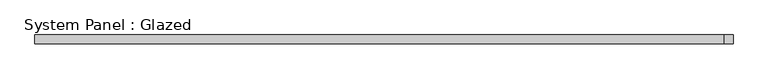
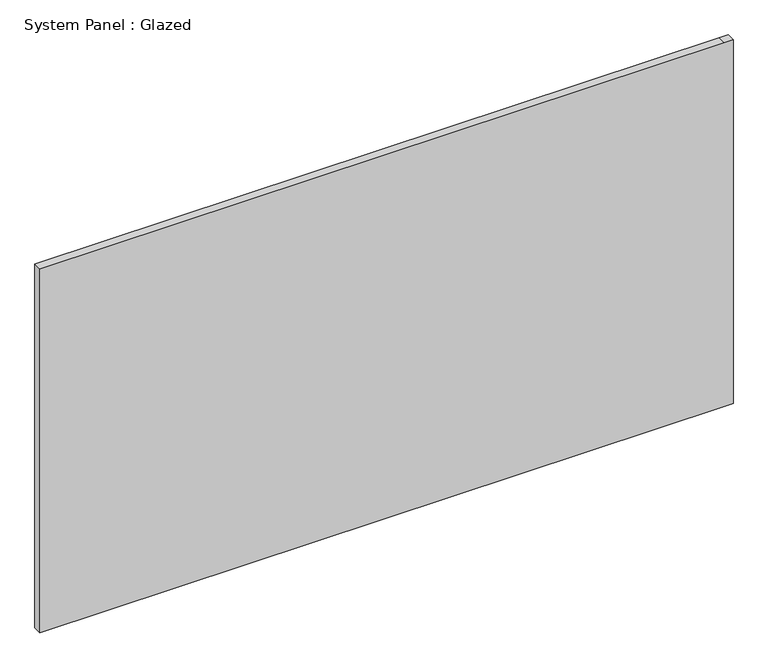
"""IFC4 building model written with IfcOpenShell, lengths in millimetres: plate geometry, System Panel : Glazed."""

from ifc_helpers import new_model, si_unit, frame, origin, place, context, project, spatial, polyline, outline, extrude, source, transform, mapped, element, save


def system_panel_glazed_d6bfc804(model_context):
    return source(origin(), model_context, "Body", "SweptSolid", [
        extrude(outline(polyline([(0.0, -1012.825), (0.0, 987.425), (0.0, 1012.825), (1123.95, 1012.825), (1123.95, 987.425), (1123.95, -1012.825), (0.0, -1012.825)])), frame((0.0, -44.45, 0.0), z_axis=(0.0, 1.0, 0.0), x_axis=(0.0, 0.0, 1.0)), (0.0, 0.0, 1.0), 25.4),
    ])


if __name__ == "__main__":
    model = new_model("IFC4")
    model_context = context("Model", 3, world=origin())
    ifc_project = project(units=[si_unit("LENGTHUNIT", "METRE", prefix="MILLI")], contexts=[model_context])
    site = spatial("IfcSite", under=ifc_project)
    building = spatial("IfcBuilding", under=site)
    placement = place(None, origin())
    system_panel_glazed_shape = system_panel_glazed_d6bfc804(model_context)
    element("IfcPlate", 1, ObjectType="System Panel : Glazed", at=placement, inside=building, context=model_context, shape_type="MappedRepresentation", body=[
        mapped(system_panel_glazed_shape, transform((0.0, 0.0, 0.0), x_axis=(1.0, 0.0, 0.0), y_axis=(0.0, 1.0, 0.0), z_axis=(0.0, 0.0, 1.0))),
    ])
    save(model, "model.ifc")

# Revit data of these elements
# Element 1 (IfcPlate, "System Panel : Glazed")
#   Materials on its faces: "Glass"
# Materials
#   "Glass": class "Glass", colour RGB 0 128 192, transparency 0.75, Cost = 0
